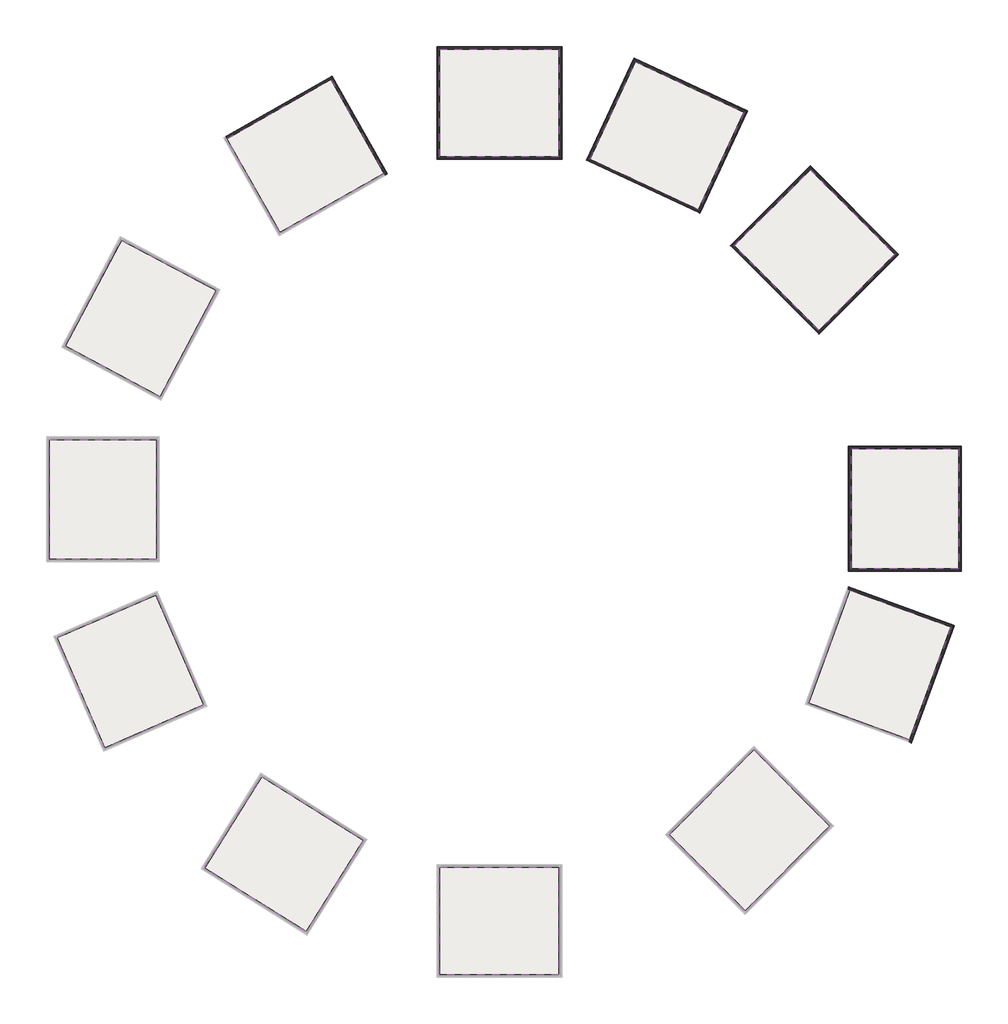
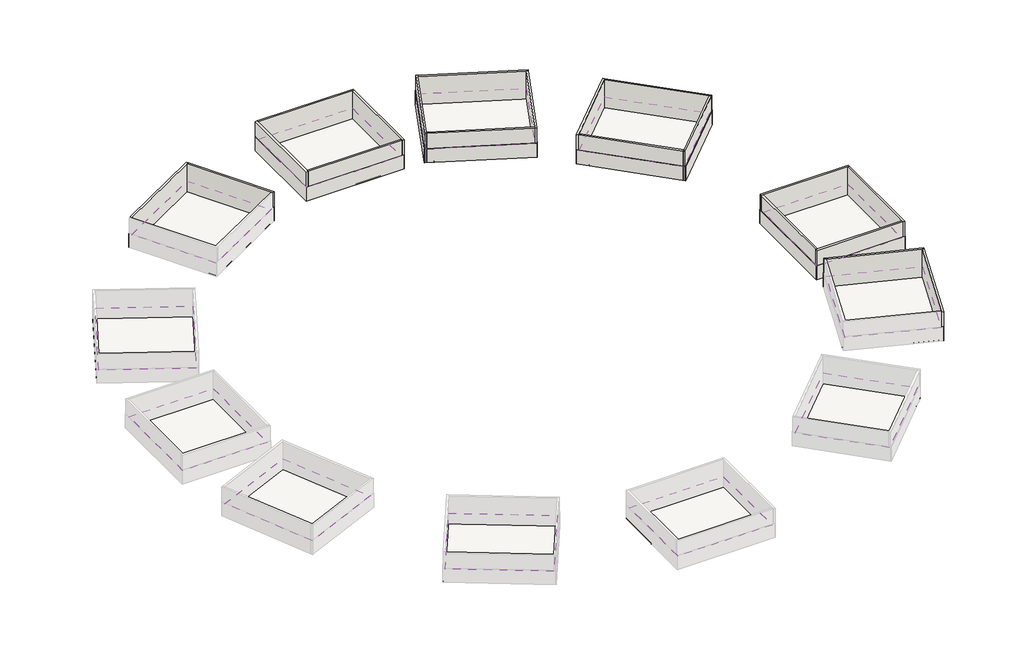
# One storey, part 2 of 2: 40 walls, 12 coverings, 12 slabs.
"""IFC4 building model written with IfcOpenShell, lengths in millimetres."""

from ifc_helpers import new_model, si_unit, frame, origin, origin_with_axes, place, context, project, spatial, polyline, outline, extrude, faceted_brep, element, save

model = new_model("IFC4")

# Units and contexts
model_context = context("Model", 3, world=origin())
ifc_project = project(units=[si_unit("LENGTHUNIT", "METRE", prefix="MILLI")], contexts=[model_context])

# Site, building, storey
site = spatial("IfcSite", under=ifc_project)
building = spatial("IfcBuilding", under=site)
storey = spatial("IfcBuildingStorey", under=building, Name="01 этаж_+0.000", Elevation=0.0)

# Coverings
placement = place(None, origin())
element("IfcCovering", 1, ObjectType="Тип 7.1_Потолок 2ГКЛ_Бирюзовый-37,5мм", at=placement, inside=storey, context=model_context, shape_type="SweptSolid", body=[
    extrude(outline(polyline([(190.0, 190.0), (190.0, 17810.0), (19810.0, 17810.0), (19810.0, 190.0), (190.0, 190.0)])), frame((0.0, 0.0, 2600.0), z_axis=(0.0, 0.0, 1.0), x_axis=(1.0, 0.0, 0.0)), (0.0, 0.0, 1.0), 37.5),
])
element("IfcCovering", 2, ObjectType="Тип 7.1_Потолок 2ГКЛ_Бирюзовый-37,5мм", at=placement, inside=storey, context=model_context, shape_type="SweptSolid", body=[
    extrude(outline(polyline([(67658.0374315, -47658.0374315), (85278.0374315, -47658.0374315), (85278.0374315, -67278.0374315), (67658.0374315, -67278.0374315), (67658.0374315, -47658.0374315)])), frame((0.0, 0.0, 2600.0), z_axis=(0.0, 0.0, 1.0), x_axis=(1.0, 0.0, 0.0)), (0.0, 0.0, 1.0), 37.5),
])
element("IfcCovering", 3, ObjectType="Тип 7.1_Потолок 2ГКЛ_Бирюзовый-37,5мм", at=placement, inside=storey, context=model_context, shape_type="SweptSolid", body=[
    extrude(outline(polyline([(19810.0, -116190.0), (19810.0, -133810.0), (190.0, -133810.0), (190.0, -116190.0), (19810.0, -116190.0)])), frame((0.0, 0.0, 2600.0), z_axis=(0.0, 0.0, 1.0), x_axis=(1.0, 0.0, 0.0)), (0.0, 0.0, 1.0), 37.5),
])
element("IfcCovering", 4, ObjectType="Тип 7.1_Потолок 2ГКЛ_Бирюзовый-37,5мм", at=placement, inside=storey, context=model_context, shape_type="SweptSolid", body=[
    extrude(outline(polyline([(-46145.4225187, -65750.266627), (-63765.4225187, -65750.266627), (-63765.4225187, -46130.266627), (-46145.4225187, -46130.266627), (-46145.4225187, -65750.266627)])), frame((0.0, 0.0, 2600.0), z_axis=(0.0, 0.0, 1.0), x_axis=(1.0, 0.0, 0.0)), (0.0, 0.0, 1.0), 37.5),
])
element("IfcCovering", 5, ObjectType="Тип 7.1_Потолок 2ГКЛ_Бирюзовый-37,5мм", at=placement, inside=storey, context=model_context, shape_type="SweptSolid", body=[
    extrude(outline(polyline([(24871.4148598, -181.3383267), (32317.9486316, 15787.8048809), (50099.7074133, 7496.0345856), (42653.1736414, -8473.108622), (24871.4148598, -181.3383267)])), frame((0.0, 0.0, 2600.0), z_axis=(0.0, 0.0, 1.0), x_axis=(1.0, 0.0, 0.0)), (0.0, 0.0, 1.0), 37.5),
])
element("IfcCovering", 6, ObjectType="Тип 7.1_Потолок 2ГКЛ_Бирюзовый-37,5мм", at=placement, inside=storey, context=model_context, shape_type="SweptSolid", body=[
    extrude(outline(polyline([(48493.2155954, -14382.134138), (60952.4370799, -1922.9126535), (74825.8721268, -15796.3477004), (62366.6506423, -28255.5691849), (48493.2155954, -14382.134138)])), frame((0.0, 0.0, 2600.0), z_axis=(0.0, 0.0, 1.0), x_axis=(1.0, 0.0, 0.0)), (0.0, 0.0, 1.0), 37.5),
])
element("IfcCovering", 7, ObjectType="Тип 7.1_Потолок 2ГКЛ_Бирюзовый-37,5мм", at=placement, inside=storey, context=model_context, shape_type="SweptSolid", body=[
    extrude(outline(polyline([(67431.6496951, -70824.335598), (83989.0336734, -76850.7305234), (77278.5984613, -95287.4997432), (60721.2144831, -89261.1048178), (67431.6496951, -70824.335598)])), frame((0.0, 0.0, 2600.0), z_axis=(0.0, 0.0, 1.0), x_axis=(1.0, 0.0, 0.0)), (0.0, 0.0, 1.0), 37.5),
])
element("IfcCovering", 8, ObjectType="Тип 7.1_Потолок 2ГКЛ_Бирюзовый-37,5мм", at=placement, inside=storey, context=model_context, shape_type="SweptSolid", body=[
    extrude(outline(polyline([(51728.6942428, -96969.0122598), (64187.9157273, -109428.2337443), (50314.4806804, -123301.6687912), (37855.2591959, -110842.4473067), (51728.6942428, -96969.0122598)])), frame((0.0, 0.0, 2600.0), z_axis=(0.0, 0.0, 1.0), x_axis=(1.0, 0.0, 0.0)), (0.0, 0.0, 1.0), 37.5),
])
element("IfcCovering", 9, ObjectType="Тип 7.1_Потолок 2ГКЛ_Бирюзовый-37,5мм", at=placement, inside=storey, context=model_context, shape_type="SweptSolid", body=[
    extrude(outline(polyline([(-12293.6410034, -111768.7013351), (-21630.8184392, -126711.3087894), (-38269.5220858, -116314.2928251), (-28932.34465, -101371.6853708), (-12293.6410034, -111768.7013351)])), frame((0.0, 0.0, 2600.0), z_axis=(0.0, 0.0, 1.0), x_axis=(1.0, 0.0, 0.0)), (0.0, 0.0, 1.0), 37.5),
])
element("IfcCovering", 10, ObjectType="Тип 7.1_Потолок 2ГКЛ_Бирюзовый-37,5мм", at=placement, inside=storey, context=model_context, shape_type="SweptSolid", body=[
    extrude(outline(polyline([(-38463.9052652, -89575.8130744), (-54622.5037758, -96601.7716689), (-62445.9605082, -78609.0530095), (-46287.3619975, -71583.094415), (-38463.9052652, -89575.8130744)])), frame((0.0, 0.0, 2600.0), z_axis=(0.0, 0.0, 1.0), x_axis=(1.0, 0.0, 0.0)), (0.0, 0.0, 1.0), 37.5),
])
element("IfcCovering", 11, ObjectType="Тип 7.1_Потолок 2ГКЛ_Бирюзовый-37,5мм", at=placement, inside=storey, context=model_context, shape_type="SweptSolid", body=[
    extrude(outline(polyline([(-45572.7204746, -39095.9018981), (-61130.2570608, -30823.8129618), (-51919.2249989, -13500.3811899), (-36361.6884127, -21772.4701262), (-45572.7204746, -39095.9018981)])), frame((0.0, 0.0, 2600.0), z_axis=(0.0, 0.0, 1.0), x_axis=(1.0, 0.0, 0.0)), (0.0, 0.0, 1.0), 37.5),
])
element("IfcCovering", 12, ObjectType="Тип 7.1_Потолок 2ГКЛ_Бирюзовый-37,5мм", at=placement, inside=storey, context=model_context, shape_type="SweptSolid", body=[
    extrude(outline(polyline([(-25945.8215879, -12171.9449727), (-34622.3247169, 3163.7223897), (-17545.9459626, 12825.072639), (-8869.4428335, -2510.5947235), (-25945.8215879, -12171.9449727)])), frame((0.0, 0.0, 2600.0), z_axis=(0.0, 0.0, 1.0), x_axis=(1.0, 0.0, 0.0)), (0.0, 0.0, 1.0), 37.5),
])

# Slabs
element("IfcSlab", 13, ObjectType="Перекрытие_Б220", at=placement, inside=storey, context=model_context, shape_type="SweptSolid", body=[
    extrude(outline(polyline([(20190.0, 18190.0), (20190.0, -190.0), (-190.0, -190.0), (-190.0, 18190.0), (20190.0, 18190.0)])), origin_with_axes(), (0.0, 0.0, 1.0), 220.0),
])
element("IfcSlab", 14, ObjectType="Перекрытие_Б220", at=placement, inside=storey, context=model_context, shape_type="SweptSolid", body=[
    extrude(outline(polyline([(85658.0374315, -67658.0374315), (67278.0374315, -67658.0374315), (67278.0374315, -47278.0374315), (85658.0374315, -47278.0374315), (85658.0374315, -67658.0374315)])), origin_with_axes(), (0.0, 0.0, 1.0), 220.0),
])
element("IfcSlab", 15, ObjectType="Перекрытие_Б220", at=placement, inside=storey, context=model_context, shape_type="SweptSolid", body=[
    extrude(outline(polyline([(-190.0, -134190.0), (-190.0, -115810.0), (20190.0, -115810.0), (20190.0, -134190.0), (-190.0, -134190.0)])), origin_with_axes(), (0.0, 0.0, 1.0), 220.0),
])
element("IfcSlab", 16, ObjectType="Перекрытие_Б220", at=placement, inside=storey, context=model_context, shape_type="SweptSolid", body=[
    extrude(outline(polyline([(-64145.4225187, -45750.266627), (-45765.4225187, -45750.266627), (-45765.4225187, -66130.266627), (-64145.4225187, -66130.266627), (-64145.4225187, -45750.266627)])), origin_with_axes(), (0.0, 0.0, 1.0), 220.0),
])
element("IfcSlab", 17, ObjectType="Перекрытие_Б220", at=placement, inside=storey, context=model_context, shape_type="SweptSolid", body=[
    extrude(outline(polyline([(50604.6993118, 7679.8366052), (42836.975661, -8978.1005205), (24366.4229612, -365.1403463), (32134.146612, 16292.7967795), (50604.6993118, 7679.8366052)])), origin_with_axes(), (0.0, 0.0, 1.0), 220.0),
])
element("IfcSlab", 18, ObjectType="Перекрытие_Б220", at=placement, inside=storey, context=model_context, shape_type="SweptSolid", body=[
    extrude(outline(polyline([(75363.2732805, -15796.3477004), (62366.6506423, -28792.9703386), (47955.8144417, -14382.134138), (60952.4370799, -1385.5114998), (75363.2732805, -15796.3477004)])), origin_with_axes(), (0.0, 0.0, 1.0), 220.0),
])
element("IfcSlab", 19, ObjectType="Перекрытие_Б220", at=placement, inside=storey, context=model_context, shape_type="SweptSolid", body=[
    extrude(outline(polyline([(77505.7140028, -95774.5505936), (60234.1636327, -89488.2203593), (67204.5341537, -70337.2847476), (84476.0845237, -76623.614982), (77505.7140028, -95774.5505936)])), origin_with_axes(), (0.0, 0.0, 1.0), 220.0),
])
element("IfcSlab", 20, ObjectType="Перекрытие_Б220", at=placement, inside=storey, context=model_context, shape_type="SweptSolid", body=[
    extrude(outline(polyline([(50314.4806804, -123839.0699449), (37317.8580422, -110842.4473067), (51728.6942428, -96431.6111061), (64725.316881, -109428.2337443), (50314.4806804, -123839.0699449)])), origin_with_axes(), (0.0, 0.0, 1.0), 220.0),
])
element("IfcSlab", 21, ObjectType="Перекрытие_Б220", at=placement, inside=storey, context=model_context, shape_type="SweptSolid", body=[
    extrude(outline(polyline([(-38793.1496827, -116435.1817812), (-29053.2336061, -100848.0577739), (-11770.0134064, -111647.812379), (-21509.929483, -127234.9363863), (-38793.1496827, -116435.1817812)])), origin_with_axes(), (0.0, 0.0, 1.0), 220.0),
])
element("IfcSlab", 22, ObjectType="Перекрытие_Б220", at=placement, inside=storey, context=model_context, shape_type="SweptSolid", body=[
    extrude(outline(polyline([(-62945.9679826, -78412.0948274), (-46090.4038154, -71083.0869405), (-37963.8977907, -89772.7712565), (-54819.4619579, -97101.7791433), (-62945.9679826, -78412.0948274)])), origin_with_axes(), (0.0, 0.0, 1.0), 220.0),
])
element("IfcSlab", 23, ObjectType="Перекрытие_Б220", at=placement, inside=storey, context=model_context, shape_type="SweptSolid", body=[
    extrude(outline(polyline([(-52076.3458903, -12986.4619107), (-35847.7691336, -21615.3492347), (-45415.5995832, -39609.8211772), (-61644.1763399, -30980.9338532), (-52076.3458903, -12986.4619107)])), origin_with_axes(), (0.0, 0.0, 1.0), 220.0),
])
element("IfcSlab", 24, ObjectType="Перекрытие_Б220", at=placement, inside=storey, context=model_context, shape_type="SweptSolid", body=[
    extrude(outline(polyline([(-17402.3317509, 13342.9287563), (-8351.5867162, -2654.2089351), (-26089.4357995, -12689.80109), (-35140.1808342, 3307.3366013), (-17402.3317509, 13342.9287563)])), origin_with_axes(), (0.0, 0.0, 1.0), 220.0),
])

# Walls
element("IfcWall", 25, ObjectType="Внутренняя_К380", at=placement, inside=storey, context=model_context, shape_type="Brep", body=[
    faceted_brep([(190.0, -190.0, 0.0), (190.0, 190.0, 0.0), (190.0, 17810.0, 0.0), (190.0, 18190.0, 0.0), (190.0, 18190.0, 6380.0), (190.0, 17810.0, 6380.0), (190.0, 190.0, 6380.0), (190.0, -190.0, 6380.0), (-190.0, -190.0, 0.0), (-190.0, -190.0, 6380.0), (-190.0, 18190.0, 6380.0), (-190.0, 18190.0, 0.0)], [[[0, 1, 2, 3, 4, 5, 6, 7]], [[8, 9, 10, 11]], [[3, 2, 1, 0, 8, 11]], [[7, 6, 5, 4, 10, 9]], [[4, 3, 11, 10]], [[0, 7, 9, 8]]]),
])
element("IfcWall", 26, ObjectType="Внутренняя_К380", at=placement, inside=storey, context=model_context, shape_type="Brep", body=[
    faceted_brep([(190.0, 17810.0, 0.0), (19810.0, 17810.0, 0.0), (20190.0, 17810.0, 0.0), (20190.0, 17810.0, 6380.0), (19810.0, 17810.0, 6380.0), (190.0, 17810.0, 6380.0), (190.0, 18190.0, 0.0), (190.0, 18190.0, 6380.0), (20190.0, 18190.0, 6380.0), (20190.0, 18190.0, 0.0)], [[[0, 1, 2, 3, 4, 5]], [[6, 7, 8, 9]], [[2, 1, 0, 6, 9]], [[5, 4, 3, 8, 7]], [[0, 5, 7, 6]], [[3, 2, 9, 8]]]),
])
element("IfcWall", 27, ObjectType="Внутренняя_К380", at=placement, inside=storey, context=model_context, shape_type="Brep", body=[
    faceted_brep([(19810.0, 17810.0, 0.0), (19810.0, 190.0, 0.0), (19810.0, -190.0, 0.0), (19810.0, -190.0, 6380.0), (19810.0, 190.0, 6380.0), (19810.0, 17810.0, 6380.0), (20190.0, 17810.0, 0.0), (20190.0, 17810.0, 6380.0), (20190.0, -190.0, 6380.0), (20190.0, -190.0, 0.0)], [[[0, 1, 2, 3, 4, 5]], [[6, 7, 8, 9]], [[2, 1, 0, 6, 9]], [[5, 4, 3, 8, 7]], [[0, 5, 7, 6]], [[3, 2, 9, 8]]]),
])
element("IfcWall", 28, ObjectType="Внутренняя_К380", at=placement, inside=storey, context=model_context, shape_type="SweptSolid", body=[
    extrude(outline(polyline([(190.0, 190.0), (19810.0, 190.0), (19810.0, -190.0), (190.0, -190.0), (190.0, 190.0)])), origin_with_axes(), (0.0, 0.0, 1.0), 6380.0),
])
element("IfcWall", 29, ObjectType="ОС-01 Окраска цвет белый 5мм", at=placement, inside=storey, context=model_context, shape_type="Brep", body=[
    faceted_brep([(-240.0, 18190.0, 0.0), (-190.0, 18190.0, 0.0), (20190.0, 18190.0, 0.0), (20240.0, 18190.0, 0.0), (20240.0, 18190.0, 3080.0), (20190.0, 18190.0, 3080.0), (-190.0, 18190.0, 3080.0), (-240.0, 18190.0, 3080.0), (-240.0, 18240.0, 0.0), (-240.0, 18240.0, 3080.0), (20240.0, 18240.0, 3080.0), (20240.0, 18240.0, 0.0)], [[[0, 1, 2, 3, 4, 5, 6, 7]], [[8, 9, 10, 11]], [[3, 2, 1, 0, 8, 11]], [[7, 6, 5, 4, 10, 9]], [[0, 7, 9, 8]], [[4, 3, 11, 10]]]),
])
element("IfcWall", 30, ObjectType="ОС-01 Окраска цвет белый 5мм", at=placement, inside=storey, context=model_context, shape_type="Brep", body=[
    faceted_brep([(-240.0, 18190.0, 0.0), (-240.0, -240.0, 0.0), (-240.0, -240.0, 3080.0), (-240.0, 18190.0, 3080.0), (-190.0, 18190.0, 0.0), (-190.0, 18190.0, 3080.0), (-190.0, -190.0, 3080.0), (-190.0, -240.0, 3080.0), (-190.0, -240.0, 0.0), (-190.0, -190.0, 0.0)], [[[0, 1, 2, 3]], [[4, 5, 6, 7, 8, 9]], [[1, 0, 4, 9, 8]], [[3, 2, 7, 6, 5]], [[0, 3, 5, 4]], [[2, 1, 8, 7]]]),
])
element("IfcWall", 31, ObjectType="ОС-01 Окраска цвет белый 5мм", at=placement, inside=storey, context=model_context, shape_type="Brep", body=[
    faceted_brep([(20190.0, 18190.0, 0.0), (20190.0, -190.0, 0.0), (20190.0, -240.0, 0.0), (20190.0, -240.0, 3080.0), (20190.0, -190.0, 3080.0), (20190.0, 18190.0, 3080.0), (20240.0, 18190.0, 0.0), (20240.0, 18190.0, 3080.0), (20240.0, -240.0, 3080.0), (20240.0, -240.0, 0.0)], [[[0, 1, 2, 3, 4, 5]], [[6, 7, 8, 9]], [[2, 1, 0, 6, 9]], [[5, 4, 3, 8, 7]], [[0, 5, 7, 6]], [[3, 2, 9, 8]]]),
])
element("IfcWall", 32, ObjectType="ОС-01 Окраска цвет белый 5мм", at=placement, inside=storey, context=model_context, shape_type="SweptSolid", body=[
    extrude(outline(polyline([(20190.0, -240.0), (-190.0, -240.0), (-190.0, -190.0), (20190.0, -190.0), (20190.0, -240.0)])), origin_with_axes(), (0.0, 0.0, 1.0), 3080.0),
])
element("IfcWall", 33, ObjectType="Внутренняя_К380", at=placement, inside=storey, context=model_context, shape_type="Brep", body=[
    faceted_brep([(67278.0374315, -47658.0374315, 0.0), (67658.0374315, -47658.0374315, 0.0), (85278.0374315, -47658.0374315, 0.0), (85658.0374315, -47658.0374315, 0.0), (85658.0374315, -47658.0374315, 6380.0), (85278.0374315, -47658.0374315, 6380.0), (67658.0374315, -47658.0374315, 6380.0), (67278.0374315, -47658.0374315, 6380.0), (67278.0374315, -47278.0374315, 0.0), (67278.0374315, -47278.0374315, 6380.0), (85658.0374315, -47278.0374315, 6380.0), (85658.0374315, -47278.0374315, 0.0)], [[[0, 1, 2, 3, 4, 5, 6, 7]], [[8, 9, 10, 11]], [[3, 2, 1, 0, 8, 11]], [[7, 6, 5, 4, 10, 9]], [[4, 3, 11, 10]], [[0, 7, 9, 8]]]),
])
element("IfcWall", 34, ObjectType="Внутренняя_К380", at=placement, inside=storey, context=model_context, shape_type="Brep", body=[
    faceted_brep([(85278.0374315, -47658.0374315, 0.0), (85278.0374315, -67278.0374315, 0.0), (85278.0374315, -67658.0374315, 0.0), (85278.0374315, -67658.0374315, 6380.0), (85278.0374315, -67278.0374315, 6380.0), (85278.0374315, -47658.0374315, 6380.0), (85658.0374315, -47658.0374315, 0.0), (85658.0374315, -47658.0374315, 6380.0), (85658.0374315, -67658.0374315, 6380.0), (85658.0374315, -67658.0374315, 0.0)], [[[0, 1, 2, 3, 4, 5]], [[6, 7, 8, 9]], [[2, 1, 0, 6, 9]], [[5, 4, 3, 8, 7]], [[0, 5, 7, 6]], [[3, 2, 9, 8]]]),
])
element("IfcWall", 35, ObjectType="Внутренняя_К380", at=placement, inside=storey, context=model_context, shape_type="Brep", body=[
    faceted_brep([(85278.0374315, -67278.0374315, 0.0), (67658.0374315, -67278.0374315, 0.0), (67278.0374315, -67278.0374315, 0.0), (67278.0374315, -67278.0374315, 6380.0), (67658.0374315, -67278.0374315, 6380.0), (85278.0374315, -67278.0374315, 6380.0), (85278.0374315, -67658.0374315, 0.0), (85278.0374315, -67658.0374315, 6380.0), (67278.0374315, -67658.0374315, 6380.0), (67278.0374315, -67658.0374315, 0.0)], [[[0, 1, 2, 3, 4, 5]], [[6, 7, 8, 9]], [[2, 1, 0, 6, 9]], [[5, 4, 3, 8, 7]], [[0, 5, 7, 6]], [[3, 2, 9, 8]]]),
])
element("IfcWall", 36, ObjectType="Внутренняя_К380", at=placement, inside=storey, context=model_context, shape_type="SweptSolid", body=[
    extrude(outline(polyline([(67658.0374315, -47658.0374315), (67658.0374315, -67278.0374315), (67278.0374315, -67278.0374315), (67278.0374315, -47658.0374315), (67658.0374315, -47658.0374315)])), origin_with_axes(), (0.0, 0.0, 1.0), 6380.0),
])
element("IfcWall", 37, ObjectType="ОС-01 Окраска цвет белый 5мм", at=placement, inside=storey, context=model_context, shape_type="Brep", body=[
    faceted_brep([(85658.0374315, -47228.0374315, 0.0), (85658.0374315, -47278.0374315, 0.0), (85658.0374315, -67658.0374315, 0.0), (85658.0374315, -67708.0374315, 0.0), (85658.0374315, -67708.0374315, 3080.0), (85658.0374315, -67658.0374315, 3080.0), (85658.0374315, -47278.0374315, 3080.0), (85658.0374315, -47228.0374315, 3080.0), (85708.0374315, -47228.0374315, 0.0), (85708.0374315, -47228.0374315, 3080.0), (85708.0374315, -67708.0374315, 3080.0), (85708.0374315, -67708.0374315, 0.0)], [[[0, 1, 2, 3, 4, 5, 6, 7]], [[8, 9, 10, 11]], [[3, 2, 1, 0, 8, 11]], [[7, 6, 5, 4, 10, 9]], [[0, 7, 9, 8]], [[4, 3, 11, 10]]]),
])
element("IfcWall", 38, ObjectType="ОС-01 Окраска цвет белый 5мм", at=placement, inside=storey, context=model_context, shape_type="Brep", body=[
    faceted_brep([(85658.0374315, -47228.0374315, 0.0), (67228.0374315, -47228.0374315, 0.0), (67228.0374315, -47228.0374315, 3080.0), (85658.0374315, -47228.0374315, 3080.0), (85658.0374315, -47278.0374315, 0.0), (85658.0374315, -47278.0374315, 3080.0), (67278.0374315, -47278.0374315, 3080.0), (67228.0374315, -47278.0374315, 3080.0), (67228.0374315, -47278.0374315, 0.0), (67278.0374315, -47278.0374315, 0.0)], [[[0, 1, 2, 3]], [[4, 5, 6, 7, 8, 9]], [[1, 0, 4, 9, 8]], [[3, 2, 7, 6, 5]], [[0, 3, 5, 4]], [[2, 1, 8, 7]]]),
])
element("IfcWall", 39, ObjectType="ОС-01 Окраска цвет белый 5мм", at=placement, inside=storey, context=model_context, shape_type="Brep", body=[
    faceted_brep([(85658.0374315, -67658.0374315, 0.0), (67278.0374315, -67658.0374315, 0.0), (67228.0374315, -67658.0374315, 0.0), (67228.0374315, -67658.0374315, 3080.0), (67278.0374315, -67658.0374315, 3080.0), (85658.0374315, -67658.0374315, 3080.0), (85658.0374315, -67708.0374315, 0.0), (85658.0374315, -67708.0374315, 3080.0), (67228.0374315, -67708.0374315, 3080.0), (67228.0374315, -67708.0374315, 0.0)], [[[0, 1, 2, 3, 4, 5]], [[6, 7, 8, 9]], [[2, 1, 0, 6, 9]], [[5, 4, 3, 8, 7]], [[0, 5, 7, 6]], [[3, 2, 9, 8]]]),
])
element("IfcWall", 40, ObjectType="ОС-01 Окраска цвет белый 5мм", at=placement, inside=storey, context=model_context, shape_type="SweptSolid", body=[
    extrude(outline(polyline([(67228.0374315, -67658.0374315), (67228.0374315, -47278.0374315), (67278.0374315, -47278.0374315), (67278.0374315, -67658.0374315), (67228.0374315, -67658.0374315)])), origin_with_axes(), (0.0, 0.0, 1.0), 3080.0),
])
element("IfcWall", 41, ObjectType="Внутренняя_К380", at=placement, inside=storey, context=model_context, shape_type="Brep", body=[
    faceted_brep([(24710.8199203, -525.7352857, 0.0), (24871.4148598, -181.3383267, 0.0), (32317.9486316, 15787.8048809, 0.0), (32478.5435711, 16132.20184, 0.0), (32478.5435711, 16132.20184, 6380.0), (32317.9486316, 15787.8048809, 6380.0), (24871.4148598, -181.3383267, 6380.0), (24710.8199203, -525.7352857, 6380.0), (24366.4229612, -365.1403463, 0.0), (24366.4229612, -365.1403463, 6380.0), (32134.146612, 16292.7967795, 6380.0), (32134.146612, 16292.7967795, 0.0)], [[[0, 1, 2, 3, 4, 5, 6, 7]], [[8, 9, 10, 11]], [[3, 2, 1, 0, 8, 11]], [[7, 6, 5, 4, 10, 9]], [[4, 3, 11, 10]], [[0, 7, 9, 8]]]),
])
element("IfcWall", 42, ObjectType="Внутренняя_К380", at=placement, inside=storey, context=model_context, shape_type="Brep", body=[
    faceted_brep([(32317.9486316, 15787.8048809, 0.0), (50099.7074133, 7496.0345856, 0.0), (50444.1043724, 7335.4396461, 0.0), (50444.1043724, 7335.4396461, 6380.0), (50099.7074133, 7496.0345856, 6380.0), (32317.9486316, 15787.8048809, 6380.0), (32478.5435711, 16132.20184, 0.0), (32478.5435711, 16132.20184, 6380.0), (50604.6993118, 7679.8366052, 6380.0), (50604.6993118, 7679.8366052, 0.0)], [[[0, 1, 2, 3, 4, 5]], [[6, 7, 8, 9]], [[2, 1, 0, 6, 9]], [[5, 4, 3, 8, 7]], [[0, 5, 7, 6]], [[3, 2, 9, 8]]]),
])
element("IfcWall", 43, ObjectType="Внутренняя_К380", at=placement, inside=storey, context=model_context, shape_type="Brep", body=[
    faceted_brep([(50099.7074133, 7496.0345856, 0.0), (42653.1736414, -8473.108622, 0.0), (42492.578702, -8817.5055811, 0.0), (42492.578702, -8817.5055811, 6380.0), (42653.1736414, -8473.108622, 6380.0), (50099.7074133, 7496.0345856, 6380.0), (50444.1043724, 7335.4396461, 0.0), (50444.1043724, 7335.4396461, 6380.0), (42836.975661, -8978.1005205, 6380.0), (42836.975661, -8978.1005205, 0.0)], [[[0, 1, 2, 3, 4, 5]], [[6, 7, 8, 9]], [[2, 1, 0, 6, 9]], [[5, 4, 3, 8, 7]], [[0, 5, 7, 6]], [[3, 2, 9, 8]]]),
])
element("IfcWall", 44, ObjectType="Внутренняя_К380", at=placement, inside=storey, context=model_context, shape_type="SweptSolid", body=[
    extrude(outline(polyline([(24871.4148598, -181.3383267), (42653.1736414, -8473.108622), (42492.578702, -8817.5055811), (24710.8199203, -525.7352857), (24871.4148598, -181.3383267)])), origin_with_axes(), (0.0, 0.0, 1.0), 6380.0),
])
element("IfcWall", 45, ObjectType="ОС-01 Окраска цвет белый 5мм", at=placement, inside=storey, context=model_context, shape_type="Brep", body=[
    faceted_brep([(32088.8312227, 16313.9276925, 0.0), (32134.146612, 16292.7967795, 0.0), (50604.6993118, 7679.8366052, 0.0), (50650.0147012, 7658.7056921, 0.0), (50650.0147012, 7658.7056921, 3080.0), (50604.6993118, 7679.8366052, 3080.0), (32134.146612, 16292.7967795, 3080.0), (32088.8312227, 16313.9276925, 3080.0), (32109.9621358, 16359.2430819, 0.0), (32109.9621358, 16359.2430819, 3080.0), (50671.1456143, 7704.0210815, 3080.0), (50671.1456143, 7704.0210815, 0.0)], [[[0, 1, 2, 3, 4, 5, 6, 7]], [[8, 9, 10, 11]], [[3, 2, 1, 0, 8, 11]], [[7, 6, 5, 4, 10, 9]], [[0, 7, 9, 8]], [[4, 3, 11, 10]]]),
])
element("IfcWall", 46, ObjectType="ОС-01 Окраска цвет белый 5мм", at=placement, inside=storey, context=model_context, shape_type="Brep", body=[
    faceted_brep([(32088.8312227, 16313.9276925, 0.0), (24299.9766588, -389.3248225, 0.0), (24299.9766588, -389.3248225, 3080.0), (32088.8312227, 16313.9276925, 3080.0), (32134.146612, 16292.7967795, 0.0), (32134.146612, 16292.7967795, 3080.0), (24366.4229612, -365.1403463, 3080.0), (24345.2920481, -410.4557356, 3080.0), (24345.2920481, -410.4557356, 0.0), (24366.4229612, -365.1403463, 0.0)], [[[0, 1, 2, 3]], [[4, 5, 6, 7, 8, 9]], [[1, 0, 4, 9, 8]], [[3, 2, 7, 6, 5]], [[0, 3, 5, 4]], [[2, 1, 8, 7]]]),
])
element("IfcWall", 47, ObjectType="ОС-01 Окраска цвет белый 5мм", at=placement, inside=storey, context=model_context, shape_type="Brep", body=[
    faceted_brep([(50604.6993118, 7679.8366052, 0.0), (42836.975661, -8978.1005205, 0.0), (42815.844748, -9023.4159099, 0.0), (42815.844748, -9023.4159099, 3080.0), (42836.975661, -8978.1005205, 3080.0), (50604.6993118, 7679.8366052, 3080.0), (50650.0147012, 7658.7056921, 0.0), (50650.0147012, 7658.7056921, 3080.0), (42861.1601373, -9044.546823, 3080.0), (42861.1601373, -9044.546823, 0.0)], [[[0, 1, 2, 3, 4, 5]], [[6, 7, 8, 9]], [[2, 1, 0, 6, 9]], [[5, 4, 3, 8, 7]], [[0, 5, 7, 6]], [[3, 2, 9, 8]]]),
])
element("IfcWall", 48, ObjectType="ОС-01 Окраска цвет белый 5мм", at=placement, inside=storey, context=model_context, shape_type="SweptSolid", body=[
    extrude(outline(polyline([(42815.844748, -9023.4159099), (24345.2920481, -410.4557356), (24366.4229612, -365.1403463), (42836.975661, -8978.1005205), (42815.844748, -9023.4159099)])), origin_with_axes(), (0.0, 0.0, 1.0), 3080.0),
])
element("IfcWall", 49, ObjectType="Внутренняя_К380", at=placement, inside=storey, context=model_context, shape_type="Brep", body=[
    faceted_brep([(48224.5150185, -14650.8347149, 0.0), (48493.2155954, -14382.134138, 0.0), (60952.4370799, -1922.9126535, 0.0), (61221.1376568, -1654.2120767, 0.0), (61221.1376568, -1654.2120767, 6380.0), (60952.4370799, -1922.9126535, 6380.0), (48493.2155954, -14382.134138, 6380.0), (48224.5150185, -14650.8347149, 6380.0), (47955.8144417, -14382.134138, 0.0), (47955.8144417, -14382.134138, 6380.0), (60952.4370799, -1385.5114998, 6380.0), (60952.4370799, -1385.5114998, 0.0)], [[[0, 1, 2, 3, 4, 5, 6, 7]], [[8, 9, 10, 11]], [[3, 2, 1, 0, 8, 11]], [[7, 6, 5, 4, 10, 9]], [[4, 3, 11, 10]], [[0, 7, 9, 8]]]),
])
element("IfcWall", 50, ObjectType="Внутренняя_К380", at=placement, inside=storey, context=model_context, shape_type="Brep", body=[
    faceted_brep([(60952.4370799, -1922.9126535, 0.0), (74825.8721268, -15796.3477004, 0.0), (75094.5727036, -16065.0482773, 0.0), (75094.5727036, -16065.0482773, 6380.0), (74825.8721268, -15796.3477004, 6380.0), (60952.4370799, -1922.9126535, 6380.0), (61221.1376568, -1654.2120767, 0.0), (61221.1376568, -1654.2120767, 6380.0), (75363.2732805, -15796.3477004, 6380.0), (75363.2732805, -15796.3477004, 0.0)], [[[0, 1, 2, 3, 4, 5]], [[6, 7, 8, 9]], [[2, 1, 0, 6, 9]], [[5, 4, 3, 8, 7]], [[0, 5, 7, 6]], [[3, 2, 9, 8]]]),
])
element("IfcWall", 51, ObjectType="Внутренняя_К380", at=placement, inside=storey, context=model_context, shape_type="Brep", body=[
    faceted_brep([(74825.8721268, -15796.3477004, 0.0), (62366.6506423, -28255.5691849, 0.0), (62097.9500654, -28524.2697618, 0.0), (62097.9500654, -28524.2697618, 6380.0), (62366.6506423, -28255.5691849, 6380.0), (74825.8721268, -15796.3477004, 6380.0), (75094.5727036, -16065.0482773, 0.0), (75094.5727036, -16065.0482773, 6380.0), (62366.6506423, -28792.9703386, 6380.0), (62366.6506423, -28792.9703386, 0.0)], [[[0, 1, 2, 3, 4, 5]], [[6, 7, 8, 9]], [[2, 1, 0, 6, 9]], [[5, 4, 3, 8, 7]], [[0, 5, 7, 6]], [[3, 2, 9, 8]]]),
])
element("IfcWall", 52, ObjectType="Внутренняя_К380", at=placement, inside=storey, context=model_context, shape_type="SweptSolid", body=[
    extrude(outline(polyline([(48493.2155954, -14382.134138), (62366.6506423, -28255.5691849), (62097.9500654, -28524.2697618), (48224.5150185, -14650.8347149), (48493.2155954, -14382.134138)])), origin_with_axes(), (0.0, 0.0, 1.0), 6380.0),
])
element("IfcWall", 53, ObjectType="ОС-01 Окраска цвет белый 5мм", at=placement, inside=storey, context=model_context, shape_type="Brep", body=[
    faceted_brep([(60917.0817408, -1350.1561608, 0.0), (60952.4370799, -1385.5114998, 0.0), (75363.2732805, -15796.3477004, 0.0), (75398.6286195, -15831.7030395, 0.0), (75398.6286195, -15831.7030395, 3080.0), (75363.2732805, -15796.3477004, 3080.0), (60952.4370799, -1385.5114998, 3080.0), (60917.0817408, -1350.1561608, 3080.0), (60952.4370799, -1314.8008217, 0.0), (60952.4370799, -1314.8008217, 3080.0), (75433.9839586, -15796.3477004, 3080.0), (75433.9839586, -15796.3477004, 0.0)], [[[0, 1, 2, 3, 4, 5, 6, 7]], [[8, 9, 10, 11]], [[3, 2, 1, 0, 8, 11]], [[7, 6, 5, 4, 10, 9]], [[0, 7, 9, 8]], [[4, 3, 11, 10]]]),
])
element("IfcWall", 54, ObjectType="ОС-01 Окраска цвет белый 5мм", at=placement, inside=storey, context=model_context, shape_type="Brep", body=[
    faceted_brep([(60917.0817408, -1350.1561608, 0.0), (47885.1037636, -14382.134138, 0.0), (47885.1037636, -14382.134138, 3080.0), (60917.0817408, -1350.1561608, 3080.0), (60952.4370799, -1385.5114998, 0.0), (60952.4370799, -1385.5114998, 3080.0), (47955.8144417, -14382.134138, 3080.0), (47920.4591026, -14417.4894771, 3080.0), (47920.4591026, -14417.4894771, 0.0), (47955.8144417, -14382.134138, 0.0)], [[[0, 1, 2, 3]], [[4, 5, 6, 7, 8, 9]], [[1, 0, 4, 9, 8]], [[3, 2, 7, 6, 5]], [[0, 3, 5, 4]], [[2, 1, 8, 7]]]),
])
element("IfcWall", 55, ObjectType="ОС-01 Окраска цвет белый 5мм", at=placement, inside=storey, context=model_context, shape_type="Brep", body=[
    faceted_brep([(75363.2732805, -15796.3477004, 0.0), (62366.6506423, -28792.9703386, 0.0), (62331.2953032, -28828.3256777, 0.0), (62331.2953032, -28828.3256777, 3080.0), (62366.6506423, -28792.9703386, 3080.0), (75363.2732805, -15796.3477004, 3080.0), (75398.6286195, -15831.7030395, 0.0), (75398.6286195, -15831.7030395, 3080.0), (62366.6506423, -28863.6810167, 3080.0), (62366.6506423, -28863.6810167, 0.0)], [[[0, 1, 2, 3, 4, 5]], [[6, 7, 8, 9]], [[2, 1, 0, 6, 9]], [[5, 4, 3, 8, 7]], [[0, 5, 7, 6]], [[3, 2, 9, 8]]]),
])
element("IfcWall", 56, ObjectType="ОС-01 Окраска цвет белый 5мм", at=placement, inside=storey, context=model_context, shape_type="SweptSolid", body=[
    extrude(outline(polyline([(62331.2953032, -28828.3256777), (47920.4591026, -14417.4894771), (47955.8144417, -14382.134138), (62366.6506423, -28792.9703386), (62331.2953032, -28828.3256777)])), origin_with_axes(), (0.0, 0.0, 1.0), 3080.0),
])
element("IfcWall", 57, ObjectType="Внутренняя_К380", at=placement, inside=storey, context=model_context, shape_type="Brep", body=[
    faceted_brep([(67074.5664992, -70694.3679435, 0.0), (67431.6496951, -70824.335598, 0.0), (83989.0336734, -76850.7305234, 0.0), (84346.1168693, -76980.6981779, 0.0), (84346.1168693, -76980.6981779, 6380.0), (83989.0336734, -76850.7305234, 6380.0), (67431.6496951, -70824.335598, 6380.0), (67074.5664992, -70694.3679435, 6380.0), (67204.5341537, -70337.2847476, 0.0), (67204.5341537, -70337.2847476, 6380.0), (84476.0845237, -76623.614982, 6380.0), (84476.0845237, -76623.614982, 0.0)], [[[0, 1, 2, 3, 4, 5, 6, 7]], [[8, 9, 10, 11]], [[3, 2, 1, 0, 8, 11]], [[7, 6, 5, 4, 10, 9]], [[4, 3, 11, 10]], [[0, 7, 9, 8]]]),
])
element("IfcWall", 58, ObjectType="Внутренняя_К380", at=placement, inside=storey, context=model_context, shape_type="Brep", body=[
    faceted_brep([(83989.0336734, -76850.7305234, 0.0), (77278.5984613, -95287.4997432, 0.0), (77148.6308069, -95644.5829391, 0.0), (77148.6308069, -95644.5829391, 6380.0), (77278.5984613, -95287.4997432, 6380.0), (83989.0336734, -76850.7305234, 6380.0), (84346.1168693, -76980.6981779, 0.0), (84346.1168693, -76980.6981779, 6380.0), (77505.7140028, -95774.5505936, 6380.0), (77505.7140028, -95774.5505936, 0.0)], [[[0, 1, 2, 3, 4, 5]], [[6, 7, 8, 9]], [[2, 1, 0, 6, 9]], [[5, 4, 3, 8, 7]], [[0, 5, 7, 6]], [[3, 2, 9, 8]]]),
])
element("IfcWall", 59, ObjectType="ОС-01 Окраска цвет белый 5мм", at=placement, inside=storey, context=model_context, shape_type="Brep", body=[
    faceted_brep([(84493.1855309, -76576.6303509, 0.0), (84476.0845237, -76623.614982, 0.0), (77505.7140028, -95774.5505936, 0.0), (77488.6129956, -95821.5352246, 0.0), (77488.6129956, -95821.5352246, 3080.0), (77505.7140028, -95774.5505936, 3080.0), (84476.0845237, -76623.614982, 3080.0), (84493.1855309, -76576.6303509, 3080.0), (84540.1701619, -76593.7313581, 0.0), (84540.1701619, -76593.7313581, 3080.0), (77535.5976266, -95838.6362318, 3080.0), (77535.5976266, -95838.6362318, 0.0)], [[[0, 1, 2, 3, 4, 5, 6, 7]], [[8, 9, 10, 11]], [[3, 2, 1, 0, 8, 11]], [[7, 6, 5, 4, 10, 9]], [[0, 7, 9, 8]], [[4, 3, 11, 10]]]),
])
element("IfcWall", 60, ObjectType="ОС-01 Окраска цвет белый 5мм", at=placement, inside=storey, context=model_context, shape_type="Brep", body=[
    faceted_brep([(84493.1855309, -76576.6303509, 0.0), (67174.6505298, -70273.1991094, 0.0), (67174.6505298, -70273.1991094, 3080.0), (84493.1855309, -76576.6303509, 3080.0), (84476.0845237, -76623.614982, 0.0), (84476.0845237, -76623.614982, 3080.0), (67204.5341537, -70337.2847476, 3080.0), (67157.5495227, -70320.1837405, 3080.0), (67157.5495227, -70320.1837405, 0.0), (67204.5341537, -70337.2847476, 0.0)], [[[0, 1, 2, 3]], [[4, 5, 6, 7, 8, 9]], [[1, 0, 4, 9, 8]], [[3, 2, 7, 6, 5]], [[0, 3, 5, 4]], [[2, 1, 8, 7]]]),
])
element("IfcWall", 61, ObjectType="Внутренняя_К380", at=placement, inside=storey, context=model_context, shape_type="Brep", body=[
    faceted_brep([(-34622.3247169, 3163.7223897, 0.0), (-17545.9459626, 12825.072639, 0.0), (-17215.2107981, 13012.1935918, 0.0), (-17215.2107981, 13012.1935918, 6380.0), (-17545.9459626, 12825.072639, 6380.0), (-34622.3247169, 3163.7223897, 6380.0), (-34809.4456697, 3494.4575542, 0.0), (-34809.4456697, 3494.4575542, 6380.0), (-17402.3317509, 13342.9287563, 6380.0), (-17402.3317509, 13342.9287563, 0.0)], [[[0, 1, 2, 3, 4, 5]], [[6, 7, 8, 9]], [[2, 1, 0, 6, 9]], [[5, 4, 3, 8, 7]], [[0, 5, 7, 6]], [[3, 2, 9, 8]]]),
])
element("IfcWall", 62, ObjectType="Внутренняя_К380", at=placement, inside=storey, context=model_context, shape_type="Brep", body=[
    faceted_brep([(-17545.9459626, 12825.072639, 0.0), (-8869.4428335, -2510.5947235, 0.0), (-8682.3218807, -2841.329888, 0.0), (-8682.3218807, -2841.329888, 6380.0), (-8869.4428335, -2510.5947235, 6380.0), (-17545.9459626, 12825.072639, 6380.0), (-17215.2107981, 13012.1935918, 0.0), (-17215.2107981, 13012.1935918, 6380.0), (-8351.5867162, -2654.2089351, 6380.0), (-8351.5867162, -2654.2089351, 0.0)], [[[0, 1, 2, 3, 4, 5]], [[6, 7, 8, 9]], [[2, 1, 0, 6, 9]], [[5, 4, 3, 8, 7]], [[0, 5, 7, 6]], [[3, 2, 9, 8]]]),
])
element("IfcWall", 63, ObjectType="ОС-01 Окраска цвет белый 5мм", at=placement, inside=storey, context=model_context, shape_type="Brep", body=[
    faceted_brep([(-35183.698619, 3282.7154233, 0.0), (-35140.1808342, 3307.3366013, 0.0), (-17402.3317509, 13342.9287563, 0.0), (-17358.8139662, 13367.5499343, 0.0), (-17358.8139662, 13367.5499343, 3080.0), (-17402.3317509, 13342.9287563, 3080.0), (-35140.1808342, 3307.3366013, 3080.0), (-35183.698619, 3282.7154233, 3080.0), (-35208.319797, 3326.2332081, 0.0), (-35208.319797, 3326.2332081, 3080.0), (-17383.4351442, 13411.0677191, 3080.0), (-17383.4351442, 13411.0677191, 0.0)], [[[0, 1, 2, 3, 4, 5, 6, 7]], [[8, 9, 10, 11]], [[3, 2, 1, 0, 8, 11]], [[7, 6, 5, 4, 10, 9]], [[0, 7, 9, 8]], [[4, 3, 11, 10]]]),
])
element("IfcWall", 64, ObjectType="ОС-01 Окраска цвет белый 5мм", at=placement, inside=storey, context=model_context, shape_type="Brep", body=[
    faceted_brep([(-17402.3317509, 13342.9287563, 0.0), (-8351.5867162, -2654.2089351, 0.0), (-8326.9655382, -2697.7267199, 0.0), (-8326.9655382, -2697.7267199, 3080.0), (-8351.5867162, -2654.2089351, 3080.0), (-17402.3317509, 13342.9287563, 3080.0), (-17358.8139662, 13367.5499343, 0.0), (-17358.8139662, 13367.5499343, 3080.0), (-8283.4477534, -2673.1055419, 3080.0), (-8283.4477534, -2673.1055419, 0.0)], [[[0, 1, 2, 3, 4, 5]], [[6, 7, 8, 9]], [[2, 1, 0, 6, 9]], [[5, 4, 3, 8, 7]], [[0, 5, 7, 6]], [[3, 2, 9, 8]]]),
])

save(model, "model.ifc")

# Revit data of these elements
# Type "Тип 7.1_Потолок 2ГКЛ_Бирюзовый-37,5мм"
#   Model = "Потолок гипсокартонный"
#   Type Comments = "Подвесной потолок из КНАУФ-листов на двухуровневом металлическом каркасе П 112.. Комплектная система КНАУФ. Финишное покрытие: Водно-дисперсионная краска DULUX 3D WHITE матовая, 2 слоя., Цвет: RAL 5021 (Бирюзовый)"
#   Description = "Подвесной потолок из КНАУФ-листов на двухуровневом металлическом каркасе П 112.. Комплектная система КНАУФ. Финишное покрытие: Водно-дисперсионная краска DULUX 3D WHITE матовая, 2 слоя., Цвет: RAL 5021 (Бирюзовый)"
#   built-in parameter 1002203 = 1 (stored number, unit not read)
#   built-in parameter 1002202 = 1 (stored number, unit not read)
#   Layers, outside or top first: 27 mm no material (function 2); 9.5 mm "Гипсокартон" (function 5); 1 mm "Окраска цвет бирюзовый" (function 5)
# Type "Перекрытие_Б220"
#   Model = "АР"
#   Function = 0
#   Layers, outside or top first: 220 mm "Бетон B20" (function 1)
# Type "Внутренняя_К380"
#   Type Mark = "рап"
#   Layers, outside or top first: 380 mm "Кирпич керамический полтнотелый(штриховка 1:50)" (function 1)
# Type "ОС-01 Окраска цвет белый 5мм"
#   Model = "Отделка стен"
#   Type Mark = "ОС-01"
#   Layers, outside or top first: 50 mm "ОС-01 Окраска цвет белый" (function 5)
# Elements 1, 2, 3, 4, 5, 6, 7, 8, 9, 10, 11, 12 (IfcCovering, "Тип 7.1_Потолок 2ГКЛ_Бирюзовый-37,5мм")
#   Height Offset From Level = 2600 mm
#   Phase Created = 1
#   Materials on its faces: "Окраска цвет бирюзовый"
# Element 13 (IfcSlab, "Перекрытие_Б220")
#   Height Offset From Level = 220 mm
#   Phase Created = 1
#   Materials on its faces: "Бетон B20"
# Element 14 (IfcSlab, "Перекрытие_Б220")
#   built-in parameter 1001955 = -1.5708 (stored number, unit not read)
#   Height Offset From Level = 220 mm
#   Phase Created = 1
#   Materials on its faces: "Бетон B20"
# Element 15 (IfcSlab, "Перекрытие_Б220")
#   built-in parameter 1001955 = 3.14159 (stored number, unit not read)
#   Height Offset From Level = 220 mm
#   Phase Created = 1
#   Materials on its faces: "Бетон B20"
# Element 16 (IfcSlab, "Перекрытие_Б220")
#   built-in parameter 1001955 = 1.5708 (stored number, unit not read)
#   Height Offset From Level = 220 mm
#   Phase Created = 1
#   Materials on its faces: "Бетон B20"
# Element 17 (IfcSlab, "Перекрытие_Б220")
#   built-in parameter 1001955 = -0.436332 (stored number, unit not read)
#   Height Offset From Level = 220 mm
#   Phase Created = 1
#   Materials on its faces: "Бетон B20"
# Element 18 (IfcSlab, "Перекрытие_Б220")
#   built-in parameter 1001955 = -0.785398 (stored number, unit not read)
#   Height Offset From Level = 220 mm
#   Phase Created = 1
#   Materials on its faces: "Бетон B20"
# Element 19 (IfcSlab, "Перекрытие_Б220")
#   built-in parameter 1001955 = -1.91986 (stored number, unit not read)
#   Height Offset From Level = 220 mm
#   Phase Created = 1
#   Materials on its faces: "Бетон B20"
# Element 20 (IfcSlab, "Перекрытие_Б220")
#   built-in parameter 1001955 = -2.35619 (stored number, unit not read)
#   Height Offset From Level = 220 mm
#   Phase Created = 1
#   Materials on its faces: "Бетон B20"
# Element 21 (IfcSlab, "Перекрытие_Б220")
#   built-in parameter 1001955 = 2.58309 (stored number, unit not read)
#   Height Offset From Level = 220 mm
#   Phase Created = 1
#   Materials on its faces: "Бетон B20"
# Element 22 (IfcSlab, "Перекрытие_Б220")
#   built-in parameter 1001955 = 1.98095 (stored number, unit not read)
#   Height Offset From Level = 220 mm
#   Phase Created = 1
#   Materials on its faces: "Бетон B20"
# Element 23 (IfcSlab, "Перекрытие_Б220")
#   built-in parameter 1001955 = 1.0821 (stored number, unit not read)
#   Height Offset From Level = 220 mm
#   Phase Created = 1
#   Materials on its faces: "Бетон B20"
# Element 24 (IfcSlab, "Перекрытие_Б220")
#   built-in parameter 1001955 = 0.514872 (stored number, unit not read)
#   Height Offset From Level = 220 mm
#   Phase Created = 1
#   Materials on its faces: "Бетон B20"
# Elements 25, 26, 27, 28, 33, 34, 35, 36, 41, 42, 43, 44, 49, 50, 51, 52, 57, 58, 61, 62 (IfcWall, "Внутренняя_К380")
#   Top Offset = -220 mm
#   Base Offset = 0 mm
#   wall height = 6380 mm
#   Phase Created = 1
#   Base Constraint = 01 этаж_+0.000
#   Top Constraint = 03 этаж_+6.600
#   Materials on its faces: "Кирпич керамический полтнотелый(штриховка 1:50)"
# Elements 29, 30, 31, 32, 37, 38, 39, 40, 45, 46, 47, 48, 53, 54, 55, 56, 59, 60, 63, 64 (IfcWall, "ОС-01 Окраска цвет белый 5мм")
#   Top Offset = -220 mm
#   Base Offset = 0 mm
#   wall height = 3080 mm
#   Phase Created = 1
#   Base Constraint = 01 этаж_+0.000
#   Top Constraint = 02 этаж_+3.300
#   Materials on its faces: "ОС-01 Окраска цвет белый"
# Materials
#   "Гипсокартон": class "Гипсокартон", colour RGB 244 244 244, transparency 0, Description = "ГКЛ для внутренней отделки", Cost = 0
#   "Окраска цвет бирюзовый": class "Отделка потолка", colour RGB 120 120 120, transparency 0, Description = "-Грунтовка\n-Чистовая шпатлевка \n-Высококачественная водоэмульсионная окраска за 2 раза Dulux Diamond Matt, цвет:  RAL 5021 (бирюзовый)", Cost = 0
#   "Бетон B20": class "Бетон", colour RGB 120 120 120, transparency 0, Manufacturer = "Альтек", Description = "Бетон, 20 МПа", Cost = 0
#   "Кирпич керамический полтнотелый(штриховка 1:50)": class "М150", colour RGB 170 100 105, transparency 0, Manufacturer = "Альтек", Description = "Керамический кирпич", Cost = 0
#   "ОС-01 Окраска цвет белый": class "Отделка стен", colour RGB 80 80 80, transparency 0, Description = "-Грунтовка\n-Черновая шпатлевка \n-Стеклохолст\n-Чистовая шпатлевка \n-Высококачественная водоэмульсионная окраска за 2 раза Dulux Diamond Matt, цвет:  RAL 9016 (белый)", Cost = 0
